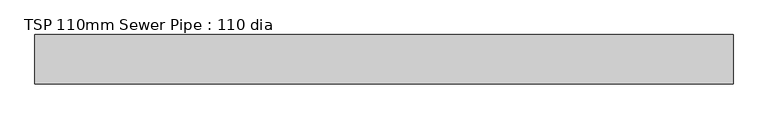
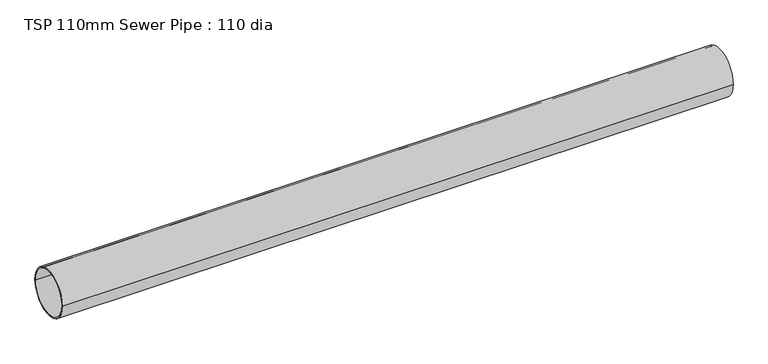
"""IFC4 building model written with IfcOpenShell, lengths in millimetres: flow terminal geometry, TSP 110mm Sewer Pipe : 110 dia."""

from ifc_helpers import new_model, si_unit, point, frame, origin, origin_2d, place, context, project, spatial, circle_curve, trimmed, segment, composite_curve, outline, extrude, source, transform, mapped, element, save


def tsp_110mm_sewer_pipe_110_dia_8147c20d(model_context):
    return source(origin(), model_context, "Body", "SweptSolid", [
        extrude(outline(composite_curve([segment(trimmed(circle_curve(origin_2d(), 55.0), [point((-55.0, 0.0))], [point((55.0, 0.0))], False, "CARTESIAN"), True, "CONTINUOUS"), segment(trimmed(circle_curve(origin_2d(), 55.0), [point((55.0, 0.0))], [point((-55.0, 0.0))], False, "CARTESIAN"), True, "CONTINUOUS")], self_intersect=False), holes=[composite_curve([segment(trimmed(circle_curve(origin_2d(), 52.0), [point((-52.0, 0.0))], [point((52.0, 0.0))], True, "CARTESIAN"), True, "CONTINUOUS"), segment(trimmed(circle_curve(origin_2d(), 52.0), [point((52.0, 0.0))], [point((-52.0, 0.0))], True, "CARTESIAN"), True, "CONTINUOUS")], self_intersect=False)]), frame((0.0, 0.0, 0.0), z_axis=(1.0, 0.0, 0.0), x_axis=(0.0, 1.0, 0.0)), (0.0, 0.0, 1.0), 1555.6349186),
    ])


if __name__ == "__main__":
    model = new_model("IFC4")
    model_context = context("Model", 3, world=origin())
    ifc_project = project(units=[si_unit("LENGTHUNIT", "METRE", prefix="MILLI")], contexts=[model_context])
    site = spatial("IfcSite", under=ifc_project)
    building = spatial("IfcBuilding", under=site)
    placement = place(None, origin())
    tsp_110mm_sewer_pipe_110_dia_shape = tsp_110mm_sewer_pipe_110_dia_8147c20d(model_context)
    element("IfcFlowTerminal", 1, ObjectType="TSP 110mm Sewer Pipe : 110 dia", at=placement, inside=building, context=model_context, shape_type="MappedRepresentation", body=[
        mapped(tsp_110mm_sewer_pipe_110_dia_shape, transform((0.0, 0.0, 0.0), x_axis=(1.0, 0.0, 0.0), y_axis=(0.0, 1.0, 0.0), z_axis=(0.0, 0.0, 1.0))),
    ])
    save(model, "model.ifc")

# Revit data of these elements
# Type "TSP 110mm Sewer Pipe : 110 dia"
#   Model = "TSP_110SWB"
#   Model = "TSP_110SWB"
#   Pipe length [instance default] = 1200 mm
#   Pipe dia = 110 mm
#   built-in parameter 1001306 [instance default] = 3.93701 (stored number, unit not read)
#   Default Elevation = 0
# Element 1 (IfcFlowTerminal, "TSP 110mm Sewer Pipe : 110 dia")
#   Pipe length = 1555.635 mm
#   built-in parameter 1001306 = 5.10379 (stored number, unit not read)
#   Materials on its faces: "Laminate, Brown, Matte"
# Materials
#   "Laminate, Brown, Matte": class "Plastic", colour RGB 128 64 0, transparency 0, Description = "Plastic Laminate - Red, Matte", Cost = 0
